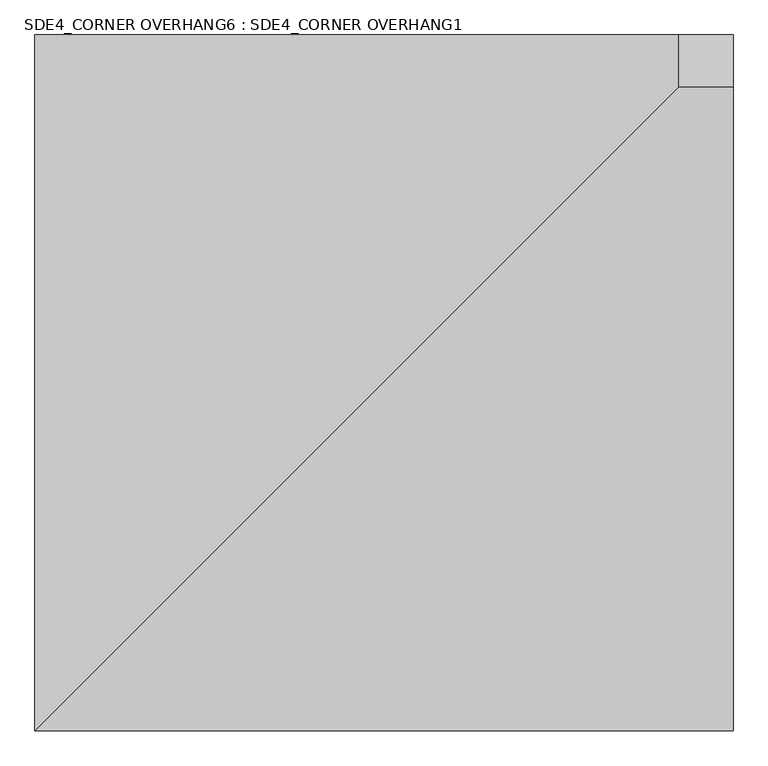
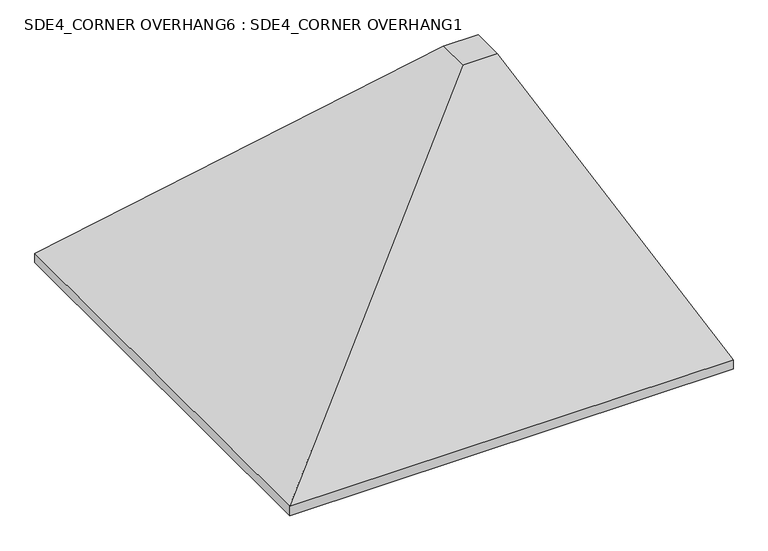
"""IFC4 building model written with IfcOpenShell, lengths in millimetres: proxy geometry, SDE4_CORNER OVERHANG6 : SDE4_CORNER OVERHANG1."""

from ifc_helpers import new_model, si_unit, origin, place, context, project, spatial, faceted_brep, source, transform, mapped, element, save


def sde4_corner_overhang6_sde4_corner_overhang1_22f262c2(model_context):
    return source(origin(), model_context, "Body", "Brep", [
        faceted_brep([(3305.0, 1190.2762268, 129960.0), (3305.0, 1190.2762268, 129920.0), (5111.5, 1190.2762268, 129920.0), (5111.5, 1190.2762268, 129960.0), (4970.0, 2990.2762268, 130270.0), (5111.5, 2990.2762268, 130270.0), (5111.5, 2990.2762268, 129920.0), (3305.0, 2990.2762268, 129920.0), (3305.0, 2990.2762268, 129960.0), (5111.5, 2855.2762268, 130270.0), (4970.0, 2855.2762268, 130270.0)], [[[0, 1, 2, 3]], [[4, 5, 6, 7, 8]], [[6, 5, 9, 3, 2]], [[2, 1, 7, 6]], [[1, 0, 8, 7]], [[4, 8, 0, 10]], [[0, 3, 9, 10]], [[5, 4, 10, 9]]]),
    ])


if __name__ == "__main__":
    model = new_model("IFC4")
    model_context = context("Model", 3, world=origin())
    ifc_project = project(units=[si_unit("LENGTHUNIT", "METRE", prefix="MILLI")], contexts=[model_context])
    site = spatial("IfcSite", under=ifc_project)
    building = spatial("IfcBuilding", under=site)
    placement = place(None, origin())
    sde4_corner_overhang6_sde4_corner_overhang1_shape = sde4_corner_overhang6_sde4_corner_overhang1_22f262c2(model_context)
    element("IfcBuildingElementProxy", 1, Name="SDE4_CORNER OVERHANG6 : SDE4_CORNER OVERHANG1", ObjectType="SDE4_CORNER OVERHANG6 : SDE4_CORNER OVERHANG1", at=placement, inside=building, context=model_context, shape_type="MappedRepresentation", body=[
        mapped(sde4_corner_overhang6_sde4_corner_overhang1_shape, transform((0.0, 0.0, 0.0), x_axis=(1.0, 0.0, 0.0), y_axis=(0.0, 1.0, 0.0), z_axis=(0.0, 0.0, 1.0))),
    ])
    save(model, "model.ifc")
